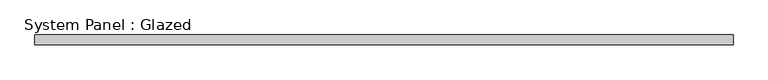
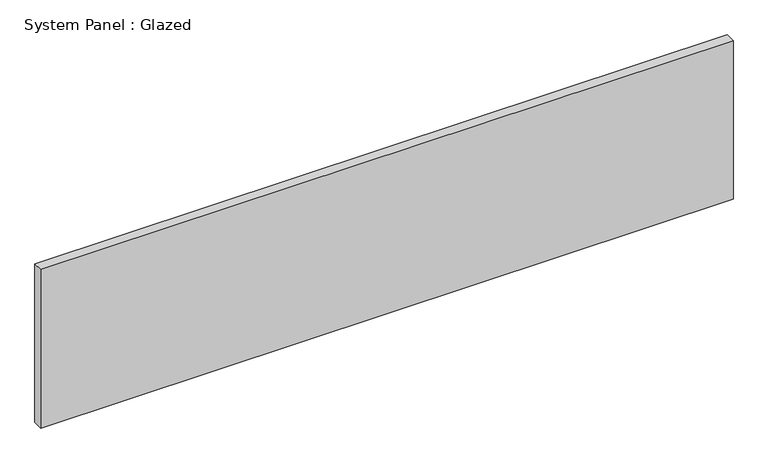
"""IFC4 building model written with IfcOpenShell, lengths in millimetres: plate geometry, System Panel : Glazed."""

from ifc_helpers import new_model, si_unit, origin, origin_with_axes, place, context, project, spatial, polyline, outline, extrude, source, transform, mapped, element, save


def system_panel_glazed_44ebf714(model_context):
    return source(origin(), model_context, "Body", "SweptSolid", [
        extrude(outline(polyline([(877.5, 24.5), (-877.5, 24.5), (-877.5, 49.5), (877.5, 49.5), (877.5, 24.5)])), origin_with_axes(), (0.0, 0.0, 1.0), 425.0),
    ])


if __name__ == "__main__":
    model = new_model("IFC4")
    model_context = context("Model", 3, world=origin())
    ifc_project = project(units=[si_unit("LENGTHUNIT", "METRE", prefix="MILLI")], contexts=[model_context])
    site = spatial("IfcSite", under=ifc_project)
    building = spatial("IfcBuilding", under=site)
    placement = place(None, origin())
    system_panel_glazed_shape = system_panel_glazed_44ebf714(model_context)
    element("IfcPlate", 1, ObjectType="System Panel : Glazed", at=placement, inside=building, context=model_context, shape_type="MappedRepresentation", body=[
        mapped(system_panel_glazed_shape, transform((0.0, 0.0, 0.0), x_axis=(1.0, 0.0, 0.0), y_axis=(0.0, 1.0, 0.0), z_axis=(0.0, 0.0, 1.0))),
    ])
    save(model, "model.ifc")

# Revit data of these elements
# Type "System Panel : Glazed"
#   Keynote = "H11"
#   Construction Type Id = "GSP4R"
#   Analytic Construction = "1/8 in Pilkington single glazing"
#   Visual Light Transmittance = 0.9
#   Solar Heat Gain Coefficient = 0.86
#   Heat Transfer Coefficient (U) = 6.7069 W/(m²·K)
# Element 1 (IfcPlate, "System Panel : Glazed")
#   Materials on its faces: "Glass"
# Materials
#   "Glass": class "Glass", colour RGB 0 128 192, transparency 0.9, Description = "Soda Lime Glass", Cost = 0
